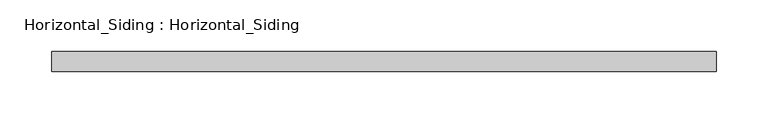
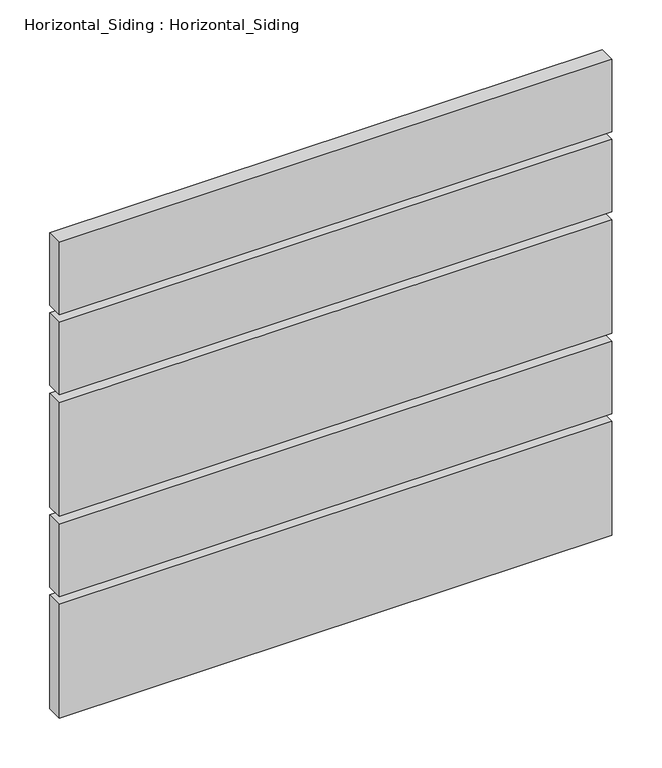
"""IFC4 building model written with IfcOpenShell, lengths in millimetres: plate geometry, Horizontal_Siding : Horizontal_Siding."""

from ifc_helpers import new_model, si_unit, frame, origin, place, context, project, spatial, polyline, outline, extrude, source, transform, mapped, element, save


def horizontal_siding_horizontal_siding_1d2bf165(model_context):
    return source(origin(), model_context, "Body", "SweptSolid", [
        extrude(outline(polyline([(320.675, -19.05), (-320.675, -19.05), (-320.675, 0.0), (320.675, 0.0), (320.675, -19.05)])), frame((0.0, 0.0, 9.525), z_axis=(0.0, 0.0, 1.0), x_axis=(1.0, 0.0, 0.0)), (0.0, 0.0, 1.0), 139.7),
        extrude(outline(polyline([(320.675, -19.05), (-320.675, -19.05), (-320.675, 0.0), (320.675, 0.0), (320.675, -19.05)])), frame((0.0, 0.0, 158.75), z_axis=(0.0, 0.0, 1.0), x_axis=(1.0, 0.0, 0.0)), (0.0, 0.0, 1.0), 88.9),
        extrude(outline(polyline([(320.675, -19.05), (-320.675, -19.05), (-320.675, 0.0), (320.675, 0.0), (320.675, -19.05)])), frame((0.0, 0.0, 257.175), z_axis=(0.0, 0.0, 1.0), x_axis=(1.0, 0.0, 0.0)), (0.0, 0.0, 1.0), 139.7),
        extrude(outline(polyline([(320.675, -19.05), (-320.675, -19.05), (-320.675, 0.0), (320.675, 0.0), (320.675, -19.05)])), frame((0.0, 0.0, 406.4), z_axis=(0.0, 0.0, 1.0), x_axis=(1.0, 0.0, 0.0)), (0.0, 0.0, 1.0), 88.9),
        extrude(outline(polyline([(320.675, -19.05), (-320.675, -19.05), (-320.675, 0.0), (320.675, 0.0), (320.675, -19.05)])), frame((0.0, 0.0, 504.825), z_axis=(0.0, 0.0, 1.0), x_axis=(1.0, 0.0, 0.0)), (0.0, 0.0, 1.0), 88.9),
    ])


if __name__ == "__main__":
    model = new_model("IFC4")
    model_context = context("Model", 3, world=origin())
    ifc_project = project(units=[si_unit("LENGTHUNIT", "METRE", prefix="MILLI")], contexts=[model_context])
    site = spatial("IfcSite", under=ifc_project)
    building = spatial("IfcBuilding", under=site)
    placement = place(None, origin())
    horizontal_siding_horizontal_siding_shape = horizontal_siding_horizontal_siding_1d2bf165(model_context)
    element("IfcPlate", 1, ObjectType="Horizontal_Siding : Horizontal_Siding", at=placement, inside=building, context=model_context, shape_type="MappedRepresentation", body=[
        mapped(horizontal_siding_horizontal_siding_shape, transform((0.0, 0.0, 0.0), x_axis=(1.0, 0.0, 0.0), y_axis=(0.0, 1.0, 0.0), z_axis=(0.0, 0.0, 1.0))),
    ])
    save(model, "model.ifc")

# Revit data of these elements
# Type "Horizontal_Siding : Horizontal_Siding"
#   Type Mark = "OUT"
#   Analytic Construction = "<None>"
#   extend = 0' - 2 3/4"
#   Width_2 = 0' - 3 1/2"
#   Width_1 = 0' - 5 1/2"
#   Gap = 0' - 0 3/8"
#   Plank Material = SLOTTED WOOD FENCE (THERMALLY MODIFIED WOOD: ARBOR WOOD)\n(EXTERIOR STAIN : PENOFIN VERDE EXT. STAIN - COLOR: CEDAR)
# Element 1 (IfcPlate, "Horizontal_Siding : Horizontal_Siding")
#   Materials on its faces: "SLOTTED WOOD FENCE (THERMALLY MODIFIED WOOD: ARBOR WOOD)\n(EXTERIOR STAIN : PENOFIN VERDE EXT. STAIN - COLOR: CEDAR)"
# Materials
#   "SLOTTED WOOD FENCE (THERMALLY MODIFIED WOOD: ARBOR WOOD)\n(EXTERIOR STAIN : PENOFIN VERDE EXT. STAIN - COLOR: CEDAR)": class "Wood", colour RGB 164 134 123, transparency 0, Description = "Pinus Echinata", Cost = 0
